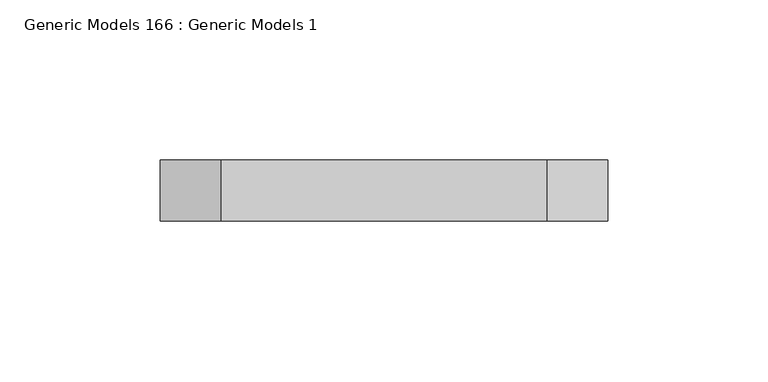
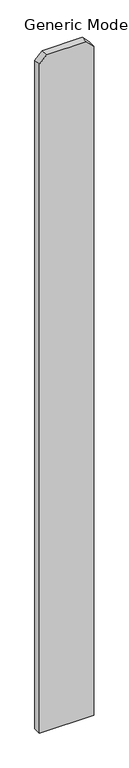
"""IFC4 building model written with IfcOpenShell, lengths in millimetres: proxy geometry, Generic Models 166 : Generic Models 1."""

import ifcopenshell
import ifcopenshell.guid

model = None  # the IFC model being written
_history = None  # IfcOwnerHistory: only IFC2X3 demands one
_inside = {}  # id of a spatial element -> (the spatial element, [elements in it])
_under = {}  # id of a project, library or spatial element -> (it, [spatial elements below it])
_declared = {}  # id of a project -> (the project, [libraries it declares])
_typed = {}  # id of a type object -> (the type object, [elements of that type])
_made_of = {}  # id of a material, layer set ... -> (it, [elements and type objects made of it])


def new_model(schema):
    """Start an empty IFC model of exactly this schema.

    Asked for "IFC4X3", IfcOpenShell would pick the latest addendum, in which some entities
    have other attributes; the version numbers below select the first issue.
    IFC2X3 requires an IfcOwnerHistory on every rooted entity: one is made here for all.
    """
    global model, _history
    if schema == "IFC4X3":
        model = ifcopenshell.file(schema_version=(4, 3, 0, 0))
    else:
        model = ifcopenshell.file(schema=schema)
    _inside.clear()
    _under.clear()
    _declared.clear()
    _typed.clear()
    _made_of.clear()
    _history = None
    if model.schema == "IFC2X3":
        org = make("IfcOrganization", Name="unknown")
        user = make(
            "IfcPersonAndOrganization",
            ThePerson=make("IfcPerson", FamilyName="unknown"),
            TheOrganization=org,
        )
        app = make(
            "IfcApplication",
            ApplicationDeveloper=org,
            Version="unknown",
            ApplicationFullName="unknown",
            ApplicationIdentifier="unknown",
        )
        _history = make(
            "IfcOwnerHistory",
            OwningUser=user,
            OwningApplication=app,
            ChangeAction="ADDED",
            CreationDate=0,
        )
    return model


def make(cls, **values):
    """One entity of the class cls with the attributes given. An attribute that is None is left unset."""
    return model.create_entity(
        cls, **{name: value for name, value in values.items() if value is not None}
    )


def rooted(cls, **values):
    """An entity with a GlobalId (a new one), such as an element, a storey or a relation."""
    return make(cls, GlobalId=ifcopenshell.guid.new(), OwnerHistory=_history, **values)


def si_unit(unit_type, name, prefix=None):
    """IfcSIUnit, for example si_unit("LENGTHUNIT", "METRE", prefix="MILLI")."""
    return make("IfcSIUnit", UnitType=unit_type, Prefix=prefix, Name=name)


def assignment(units):
    """IfcUnitAssignment: the units of a project."""
    return None if units is None else make("IfcUnitAssignment", Units=units)


def point(xyz):
    """IfcCartesianPoint."""
    return None if xyz is None else make("IfcCartesianPoint", Coordinates=xyz)


def direction(xyz):
    """IfcDirection."""
    return None if xyz is None else make("IfcDirection", DirectionRatios=xyz)


def frame(location, z_axis=None, x_axis=None):
    """IfcAxis2Placement3D, a coordinate frame: its origin and axes. An axis left out is left unset."""
    return make(
        "IfcAxis2Placement3D",
        Location=point(location),
        Axis=direction(z_axis),
        RefDirection=direction(x_axis),
    )


def origin():
    """The frame at (0, 0, 0) with its axes left unset."""
    return frame((0.0, 0.0, 0.0))


def place(relative_to, where):
    """IfcLocalPlacement: puts the frame where relative to a parent placement (None: the world)."""
    return make(
        "IfcLocalPlacement", PlacementRelTo=relative_to, RelativePlacement=where
    )


def context(
    kind, dimensions, precision=None, world=None, true_north=None, identifier=None
):
    """IfcGeometricRepresentationContext, for example the 3D "Model" context."""
    return make(
        "IfcGeometricRepresentationContext",
        ContextIdentifier=identifier,
        ContextType=kind,
        CoordinateSpaceDimension=dimensions,
        Precision=precision,
        WorldCoordinateSystem=world,
        TrueNorth=true_north,
    )


def project(units=None, contexts=None):
    """IfcProject with its units and contexts."""
    return rooted(
        "IfcProject",
        Name="project",
        RepresentationContexts=contexts,
        UnitsInContext=assignment(units),
    )


def spatial(cls, under=None, at=None, **own):
    """A site, building, storey or space (cls), placed at a placement, below another one or the project."""
    s = rooted(cls, ObjectPlacement=at, **own)
    if under is not None:
        _under.setdefault(under.id(), (under, []))[1].append(s)
    return s


def polyline(points):
    """IfcPolyline through the points."""
    return make("IfcPolyline", Points=[point(p) for p in points])


def outline(outer, holes=None, kind="AREA"):
    """IfcArbitraryClosedProfileDef: a profile drawn as a closed curve; with holes, ...WithVoids."""
    if holes is None:
        return make("IfcArbitraryClosedProfileDef", ProfileType=kind, OuterCurve=outer)
    return make(
        "IfcArbitraryProfileDefWithVoids",
        ProfileType=kind,
        OuterCurve=outer,
        InnerCurves=holes,
    )


def extrude(swept, where, along, depth):
    """IfcExtrudedAreaSolid: the profile swept, set in the frame where, extruded along a direction by depth."""
    return make(
        "IfcExtrudedAreaSolid",
        SweptArea=swept,
        Position=where,
        ExtrudedDirection=direction(along),
        Depth=depth,
    )


def shape(context_of_items, identifier, shape_type, items):
    """IfcShapeRepresentation: the items that make up one representation, for example the "Body"."""
    return make(
        "IfcShapeRepresentation",
        ContextOfItems=context_of_items,
        RepresentationIdentifier=identifier,
        RepresentationType=shape_type,
        Items=items,
    )


def source(mapping_origin, context_of_items, identifier, shape_type, items):
    """IfcRepresentationMap: a shape defined once, which mapped items show again and again."""
    return make(
        "IfcRepresentationMap",
        MappingOrigin=mapping_origin,
        MappedRepresentation=shape(context_of_items, identifier, shape_type, items),
    )


def transform(
    local_origin,
    x_axis=None,
    y_axis=None,
    z_axis=None,
    scale=None,
    scale2=None,
    scale3=None,
    uniform=True,
):
    """IfcCartesianTransformationOperator3D, or its non-uniform kind. x_axis, y_axis, z_axis: its Axis1, 2, 3."""
    if uniform:
        return make(
            "IfcCartesianTransformationOperator3D",
            Axis1=direction(x_axis),
            Axis2=direction(y_axis),
            LocalOrigin=point(local_origin),
            Scale=scale,
            Axis3=direction(z_axis),
        )
    return make(
        "IfcCartesianTransformationOperator3DnonUniform",
        Axis1=direction(x_axis),
        Axis2=direction(y_axis),
        LocalOrigin=point(local_origin),
        Scale=scale,
        Axis3=direction(z_axis),
        Scale2=scale2,
        Scale3=scale3,
    )


def mapped(mapping_source, mapping_target):
    """IfcMappedItem: shows the shape of a source again, moved by a transform."""
    return make(
        "IfcMappedItem", MappingSource=mapping_source, MappingTarget=mapping_target
    )


def made_of(thing, what):
    """Note that an element or type object is made of a material, layer set ...; save() writes the relation."""
    if what is not None:
        _made_of.setdefault(what.id(), (what, []))[1].append(thing)
    return thing


def element(
    cls,
    number,
    at=None,
    inside=None,
    cuts=None,
    type_object=None,
    material=None,
    context=None,
    identifier="Body",
    shape_type=None,
    held_by="IfcProductDefinitionShape",
    body=None,
    shapes=None,
    **own,
):
    """One element of the class cls, such as IfcWall. Its Tag is "e" and its number.

    at: its placement. inside: the storey or other place that contains it. cuts: it is an
    opening in that element (IfcRelVoidsElement). A single representation is given by context,
    identifier, shape_type and body (its items); several are given by shapes. held_by: the class
    of the entity that holds the representations. save() writes the other relations.
    """
    e = rooted(cls, Tag="e%d" % number, ObjectPlacement=at, **own)
    if body is not None:
        shapes = [shape(context, identifier, shape_type, body)]
    if shapes is not None:
        e.Representation = make(held_by, Representations=shapes)
    if inside is not None:
        _inside.setdefault(inside.id(), (inside, []))[1].append(e)
    if cuts is not None:
        rooted(
            "IfcRelVoidsElement", RelatingBuildingElement=cuts, RelatedOpeningElement=e
        )
    if type_object is not None:
        _typed.setdefault(type_object.id(), (type_object, []))[1].append(e)
    return made_of(e, material)


def aggregate(whole, parts):
    """IfcRelAggregates: a whole, such as a stair, and the parts it consists of."""
    return rooted("IfcRelAggregates", RelatingObject=whole, RelatedObjects=parts)


def save(model, path):
    """Write the relations noted so far, then the file.

    IfcRelAggregates (storeys below a building ...), IfcRelContainedInSpatialStructure (elements
    in a storey), IfcRelDefinesByType, IfcRelAssociatesMaterial and IfcRelDeclares: one each for
    every whole, place, type object, material and project.
    """
    for whole, parts in _under.values():
        aggregate(whole, parts)
    for where, things in _inside.values():
        rooted(
            "IfcRelContainedInSpatialStructure",
            RelatedElements=things,
            RelatingStructure=where,
        )
    for kind, things in _typed.values():
        rooted("IfcRelDefinesByType", RelatedObjects=things, RelatingType=kind)
    for what, things in _made_of.values():
        rooted("IfcRelAssociatesMaterial", RelatedObjects=things, RelatingMaterial=what)
    for by, libraries in _declared.values():
        rooted("IfcRelDeclares", RelatingContext=by, RelatedDefinitions=libraries)
    model.write(path)


def generic_models_166_generic_models_1_bb9aeded(model_context):
    return source(origin(), model_context, "Body", "SweptSolid", [
        extrude(outline(polyline([(76.2, 55294.2125), (1885.95, 55294.2125), (1905.0, 55275.1625), (1905.0, 55173.5625), (1885.95, 55154.5125), (76.2, 55154.5125), (76.2, 55294.2125)])), frame((0.0, 547.6875, 0.0), z_axis=(0.0, 1.0, 0.0), x_axis=(0.0, 0.0, 1.0)), (0.0, 0.0, 1.0), 19.05),
    ])


if __name__ == "__main__":
    model = new_model("IFC4")
    model_context = context("Model", 3, world=origin())
    ifc_project = project(units=[si_unit("LENGTHUNIT", "METRE", prefix="MILLI")], contexts=[model_context])
    site = spatial("IfcSite", under=ifc_project)
    building = spatial("IfcBuilding", under=site)
    placement = place(None, origin())
    generic_models_166_generic_models_1_shape = generic_models_166_generic_models_1_bb9aeded(model_context)
    element("IfcBuildingElementProxy", 1, Name="Generic Models 166 : Generic Models 1", ObjectType="Generic Models 166 : Generic Models 1", at=placement, inside=building, context=model_context, shape_type="MappedRepresentation", body=[
        mapped(generic_models_166_generic_models_1_shape, transform((0.0, 0.0, 0.0), x_axis=(1.0, 0.0, 0.0), y_axis=(0.0, 1.0, 0.0), z_axis=(0.0, 0.0, 1.0))),
    ])
    save(model, "model.ifc")

# Revit data of these elements
# Element 1 (IfcBuildingElementProxy, "Generic Models 166 : Generic Models 1")
#   Materials on its faces: "VERTICAL 1X6 CEDAR PLANKS W/ CLEAR WOOD SEALER"
# Materials
#   "VERTICAL 1X6 CEDAR PLANKS W/ CLEAR WOOD SEALER": class "Wood", colour RGB 234 198 147, transparency 0, Description = "Pinus Echinata", Cost = 0
